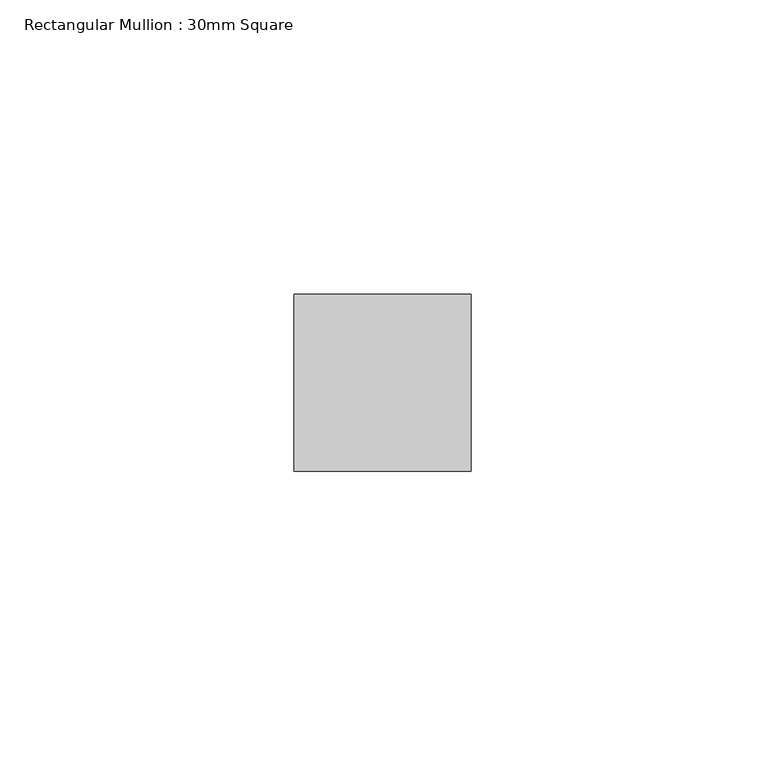
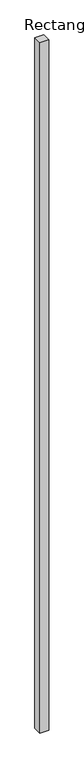
"""IFC4 building model written with IfcOpenShell, lengths in millimetres: member geometry, Rectangular Mullion : 30mm Square."""

import ifcopenshell
import ifcopenshell.guid

model = None  # the IFC model being written
_history = None  # IfcOwnerHistory: only IFC2X3 demands one
_inside = {}  # id of a spatial element -> (the spatial element, [elements in it])
_under = {}  # id of a project, library or spatial element -> (it, [spatial elements below it])
_declared = {}  # id of a project -> (the project, [libraries it declares])
_typed = {}  # id of a type object -> (the type object, [elements of that type])
_made_of = {}  # id of a material, layer set ... -> (it, [elements and type objects made of it])


def new_model(schema):
    """Start an empty IFC model of exactly this schema.

    Asked for "IFC4X3", IfcOpenShell would pick the latest addendum, in which some entities
    have other attributes; the version numbers below select the first issue.
    IFC2X3 requires an IfcOwnerHistory on every rooted entity: one is made here for all.
    """
    global model, _history
    if schema == "IFC4X3":
        model = ifcopenshell.file(schema_version=(4, 3, 0, 0))
    else:
        model = ifcopenshell.file(schema=schema)
    _inside.clear()
    _under.clear()
    _declared.clear()
    _typed.clear()
    _made_of.clear()
    _history = None
    if model.schema == "IFC2X3":
        org = make("IfcOrganization", Name="unknown")
        user = make(
            "IfcPersonAndOrganization",
            ThePerson=make("IfcPerson", FamilyName="unknown"),
            TheOrganization=org,
        )
        app = make(
            "IfcApplication",
            ApplicationDeveloper=org,
            Version="unknown",
            ApplicationFullName="unknown",
            ApplicationIdentifier="unknown",
        )
        _history = make(
            "IfcOwnerHistory",
            OwningUser=user,
            OwningApplication=app,
            ChangeAction="ADDED",
            CreationDate=0,
        )
    return model


def make(cls, **values):
    """One entity of the class cls with the attributes given. An attribute that is None is left unset."""
    return model.create_entity(
        cls, **{name: value for name, value in values.items() if value is not None}
    )


def rooted(cls, **values):
    """An entity with a GlobalId (a new one), such as an element, a storey or a relation."""
    return make(cls, GlobalId=ifcopenshell.guid.new(), OwnerHistory=_history, **values)


def si_unit(unit_type, name, prefix=None):
    """IfcSIUnit, for example si_unit("LENGTHUNIT", "METRE", prefix="MILLI")."""
    return make("IfcSIUnit", UnitType=unit_type, Prefix=prefix, Name=name)


def assignment(units):
    """IfcUnitAssignment: the units of a project."""
    return None if units is None else make("IfcUnitAssignment", Units=units)


def point(xyz):
    """IfcCartesianPoint."""
    return None if xyz is None else make("IfcCartesianPoint", Coordinates=xyz)


def direction(xyz):
    """IfcDirection."""
    return None if xyz is None else make("IfcDirection", DirectionRatios=xyz)


def frame(location, z_axis=None, x_axis=None):
    """IfcAxis2Placement3D, a coordinate frame: its origin and axes. An axis left out is left unset."""
    return make(
        "IfcAxis2Placement3D",
        Location=point(location),
        Axis=direction(z_axis),
        RefDirection=direction(x_axis),
    )


def origin():
    """The frame at (0, 0, 0) with its axes left unset."""
    return frame((0.0, 0.0, 0.0))


def place(relative_to, where):
    """IfcLocalPlacement: puts the frame where relative to a parent placement (None: the world)."""
    return make(
        "IfcLocalPlacement", PlacementRelTo=relative_to, RelativePlacement=where
    )


def context(
    kind, dimensions, precision=None, world=None, true_north=None, identifier=None
):
    """IfcGeometricRepresentationContext, for example the 3D "Model" context."""
    return make(
        "IfcGeometricRepresentationContext",
        ContextIdentifier=identifier,
        ContextType=kind,
        CoordinateSpaceDimension=dimensions,
        Precision=precision,
        WorldCoordinateSystem=world,
        TrueNorth=true_north,
    )


def project(units=None, contexts=None):
    """IfcProject with its units and contexts."""
    return rooted(
        "IfcProject",
        Name="project",
        RepresentationContexts=contexts,
        UnitsInContext=assignment(units),
    )


def spatial(cls, under=None, at=None, **own):
    """A site, building, storey or space (cls), placed at a placement, below another one or the project."""
    s = rooted(cls, ObjectPlacement=at, **own)
    if under is not None:
        _under.setdefault(under.id(), (under, []))[1].append(s)
    return s


def polyline(points):
    """IfcPolyline through the points."""
    return make("IfcPolyline", Points=[point(p) for p in points])


def outline(outer, holes=None, kind="AREA"):
    """IfcArbitraryClosedProfileDef: a profile drawn as a closed curve; with holes, ...WithVoids."""
    if holes is None:
        return make("IfcArbitraryClosedProfileDef", ProfileType=kind, OuterCurve=outer)
    return make(
        "IfcArbitraryProfileDefWithVoids",
        ProfileType=kind,
        OuterCurve=outer,
        InnerCurves=holes,
    )


def extrude(swept, where, along, depth):
    """IfcExtrudedAreaSolid: the profile swept, set in the frame where, extruded along a direction by depth."""
    return make(
        "IfcExtrudedAreaSolid",
        SweptArea=swept,
        Position=where,
        ExtrudedDirection=direction(along),
        Depth=depth,
    )


def shape(context_of_items, identifier, shape_type, items):
    """IfcShapeRepresentation: the items that make up one representation, for example the "Body"."""
    return make(
        "IfcShapeRepresentation",
        ContextOfItems=context_of_items,
        RepresentationIdentifier=identifier,
        RepresentationType=shape_type,
        Items=items,
    )


def source(mapping_origin, context_of_items, identifier, shape_type, items):
    """IfcRepresentationMap: a shape defined once, which mapped items show again and again."""
    return make(
        "IfcRepresentationMap",
        MappingOrigin=mapping_origin,
        MappedRepresentation=shape(context_of_items, identifier, shape_type, items),
    )


def transform(
    local_origin,
    x_axis=None,
    y_axis=None,
    z_axis=None,
    scale=None,
    scale2=None,
    scale3=None,
    uniform=True,
):
    """IfcCartesianTransformationOperator3D, or its non-uniform kind. x_axis, y_axis, z_axis: its Axis1, 2, 3."""
    if uniform:
        return make(
            "IfcCartesianTransformationOperator3D",
            Axis1=direction(x_axis),
            Axis2=direction(y_axis),
            LocalOrigin=point(local_origin),
            Scale=scale,
            Axis3=direction(z_axis),
        )
    return make(
        "IfcCartesianTransformationOperator3DnonUniform",
        Axis1=direction(x_axis),
        Axis2=direction(y_axis),
        LocalOrigin=point(local_origin),
        Scale=scale,
        Axis3=direction(z_axis),
        Scale2=scale2,
        Scale3=scale3,
    )


def mapped(mapping_source, mapping_target):
    """IfcMappedItem: shows the shape of a source again, moved by a transform."""
    return make(
        "IfcMappedItem", MappingSource=mapping_source, MappingTarget=mapping_target
    )


def made_of(thing, what):
    """Note that an element or type object is made of a material, layer set ...; save() writes the relation."""
    if what is not None:
        _made_of.setdefault(what.id(), (what, []))[1].append(thing)
    return thing


def element(
    cls,
    number,
    at=None,
    inside=None,
    cuts=None,
    type_object=None,
    material=None,
    context=None,
    identifier="Body",
    shape_type=None,
    held_by="IfcProductDefinitionShape",
    body=None,
    shapes=None,
    **own,
):
    """One element of the class cls, such as IfcWall. Its Tag is "e" and its number.

    at: its placement. inside: the storey or other place that contains it. cuts: it is an
    opening in that element (IfcRelVoidsElement). A single representation is given by context,
    identifier, shape_type and body (its items); several are given by shapes. held_by: the class
    of the entity that holds the representations. save() writes the other relations.
    """
    e = rooted(cls, Tag="e%d" % number, ObjectPlacement=at, **own)
    if body is not None:
        shapes = [shape(context, identifier, shape_type, body)]
    if shapes is not None:
        e.Representation = make(held_by, Representations=shapes)
    if inside is not None:
        _inside.setdefault(inside.id(), (inside, []))[1].append(e)
    if cuts is not None:
        rooted(
            "IfcRelVoidsElement", RelatingBuildingElement=cuts, RelatedOpeningElement=e
        )
    if type_object is not None:
        _typed.setdefault(type_object.id(), (type_object, []))[1].append(e)
    return made_of(e, material)


def aggregate(whole, parts):
    """IfcRelAggregates: a whole, such as a stair, and the parts it consists of."""
    return rooted("IfcRelAggregates", RelatingObject=whole, RelatedObjects=parts)


def save(model, path):
    """Write the relations noted so far, then the file.

    IfcRelAggregates (storeys below a building ...), IfcRelContainedInSpatialStructure (elements
    in a storey), IfcRelDefinesByType, IfcRelAssociatesMaterial and IfcRelDeclares: one each for
    every whole, place, type object, material and project.
    """
    for whole, parts in _under.values():
        aggregate(whole, parts)
    for where, things in _inside.values():
        rooted(
            "IfcRelContainedInSpatialStructure",
            RelatedElements=things,
            RelatingStructure=where,
        )
    for kind, things in _typed.values():
        rooted("IfcRelDefinesByType", RelatedObjects=things, RelatingType=kind)
    for what, things in _made_of.values():
        rooted("IfcRelAssociatesMaterial", RelatedObjects=things, RelatingMaterial=what)
    for by, libraries in _declared.values():
        rooted("IfcRelDeclares", RelatingContext=by, RelatedDefinitions=libraries)
    model.write(path)


def rectangular_mullion_30mm_square_17cee0f7(model_context):
    return source(origin(), model_context, "Body", "SweptSolid", [
        extrude(outline(polyline([(15.0, 15.0), (15.0, -15.0), (-15.0, -15.0), (-15.0, 15.0), (15.0, 15.0)])), frame((0.0, 0.0, -2506.1453827), z_axis=(0.0, 0.0, 1.0), x_axis=(1.0, 0.0, 0.0)), (0.0, 0.0, 1.0), 2506.1453827),
    ])


if __name__ == "__main__":
    model = new_model("IFC4")
    model_context = context("Model", 3, world=origin())
    ifc_project = project(units=[si_unit("LENGTHUNIT", "METRE", prefix="MILLI")], contexts=[model_context])
    site = spatial("IfcSite", under=ifc_project)
    building = spatial("IfcBuilding", under=site)
    placement = place(None, origin())
    rectangular_mullion_30mm_square_shape = rectangular_mullion_30mm_square_17cee0f7(model_context)
    element("IfcMember", 1, ObjectType="Rectangular Mullion : 30mm Square", at=placement, inside=building, context=model_context, shape_type="MappedRepresentation", body=[
        mapped(rectangular_mullion_30mm_square_shape, transform((0.0, 0.0, 0.0), x_axis=(1.0, 0.0, 0.0), y_axis=(0.0, 1.0, 0.0), z_axis=(0.0, 0.0, 1.0))),
    ])
    save(model, "model.ifc")

# Revit data of these elements
# Type "Rectangular Mullion : 30mm Square"
#   built-in parameter 1007304 = 0.0984252 (stored number, unit not read)
#   built-in parameter 1007301 = 0.0492126 (stored number, unit not read)
#   built-in parameter 1007300 = 0.0492126 (stored number, unit not read)
# Element 1 (IfcMember, "Rectangular Mullion : 30mm Square")
#   Materials on its faces: "Aluminum"
# Materials
#   "Aluminum": class "Metal", colour RGB 244 244 244, transparency 0, Description = "Aluminum 6061", Cost = 0
